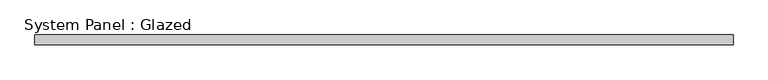
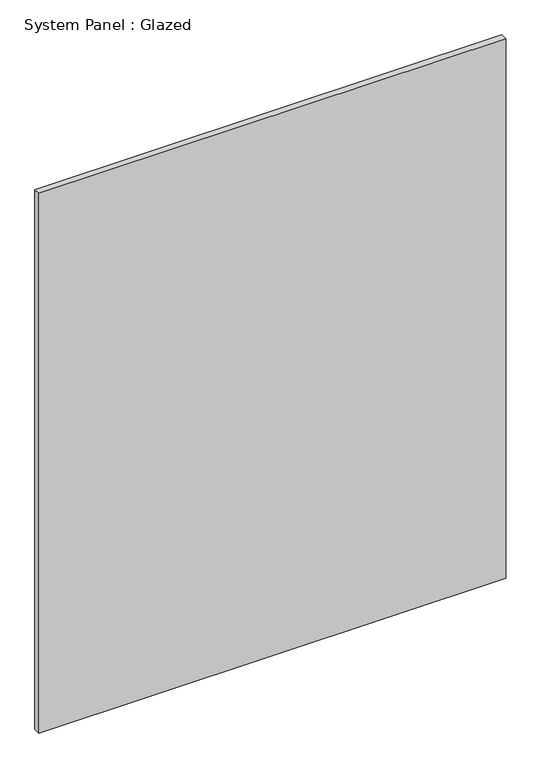
"""IFC4 building model written with IfcOpenShell, lengths in millimetres: plate geometry, System Panel : Glazed."""

import ifcopenshell
import ifcopenshell.guid

model = None  # the IFC model being written
_history = None  # IfcOwnerHistory: only IFC2X3 demands one
_inside = {}  # id of a spatial element -> (the spatial element, [elements in it])
_under = {}  # id of a project, library or spatial element -> (it, [spatial elements below it])
_declared = {}  # id of a project -> (the project, [libraries it declares])
_typed = {}  # id of a type object -> (the type object, [elements of that type])
_made_of = {}  # id of a material, layer set ... -> (it, [elements and type objects made of it])


def new_model(schema):
    """Start an empty IFC model of exactly this schema.

    Asked for "IFC4X3", IfcOpenShell would pick the latest addendum, in which some entities
    have other attributes; the version numbers below select the first issue.
    IFC2X3 requires an IfcOwnerHistory on every rooted entity: one is made here for all.
    """
    global model, _history
    if schema == "IFC4X3":
        model = ifcopenshell.file(schema_version=(4, 3, 0, 0))
    else:
        model = ifcopenshell.file(schema=schema)
    _inside.clear()
    _under.clear()
    _declared.clear()
    _typed.clear()
    _made_of.clear()
    _history = None
    if model.schema == "IFC2X3":
        org = make("IfcOrganization", Name="unknown")
        user = make(
            "IfcPersonAndOrganization",
            ThePerson=make("IfcPerson", FamilyName="unknown"),
            TheOrganization=org,
        )
        app = make(
            "IfcApplication",
            ApplicationDeveloper=org,
            Version="unknown",
            ApplicationFullName="unknown",
            ApplicationIdentifier="unknown",
        )
        _history = make(
            "IfcOwnerHistory",
            OwningUser=user,
            OwningApplication=app,
            ChangeAction="ADDED",
            CreationDate=0,
        )
    return model


def make(cls, **values):
    """One entity of the class cls with the attributes given. An attribute that is None is left unset."""
    return model.create_entity(
        cls, **{name: value for name, value in values.items() if value is not None}
    )


def rooted(cls, **values):
    """An entity with a GlobalId (a new one), such as an element, a storey or a relation."""
    return make(cls, GlobalId=ifcopenshell.guid.new(), OwnerHistory=_history, **values)


def si_unit(unit_type, name, prefix=None):
    """IfcSIUnit, for example si_unit("LENGTHUNIT", "METRE", prefix="MILLI")."""
    return make("IfcSIUnit", UnitType=unit_type, Prefix=prefix, Name=name)


def assignment(units):
    """IfcUnitAssignment: the units of a project."""
    return None if units is None else make("IfcUnitAssignment", Units=units)


def point(xyz):
    """IfcCartesianPoint."""
    return None if xyz is None else make("IfcCartesianPoint", Coordinates=xyz)


def direction(xyz):
    """IfcDirection."""
    return None if xyz is None else make("IfcDirection", DirectionRatios=xyz)


def frame(location, z_axis=None, x_axis=None):
    """IfcAxis2Placement3D, a coordinate frame: its origin and axes. An axis left out is left unset."""
    return make(
        "IfcAxis2Placement3D",
        Location=point(location),
        Axis=direction(z_axis),
        RefDirection=direction(x_axis),
    )


def origin():
    """The frame at (0, 0, 0) with its axes left unset."""
    return frame((0.0, 0.0, 0.0))


def origin_with_axes():
    """The frame at (0, 0, 0) with the z axis (0, 0, 1) and the x axis (1, 0, 0) written out."""
    return frame((0.0, 0.0, 0.0), z_axis=(0.0, 0.0, 1.0), x_axis=(1.0, 0.0, 0.0))


def place(relative_to, where):
    """IfcLocalPlacement: puts the frame where relative to a parent placement (None: the world)."""
    return make(
        "IfcLocalPlacement", PlacementRelTo=relative_to, RelativePlacement=where
    )


def context(
    kind, dimensions, precision=None, world=None, true_north=None, identifier=None
):
    """IfcGeometricRepresentationContext, for example the 3D "Model" context."""
    return make(
        "IfcGeometricRepresentationContext",
        ContextIdentifier=identifier,
        ContextType=kind,
        CoordinateSpaceDimension=dimensions,
        Precision=precision,
        WorldCoordinateSystem=world,
        TrueNorth=true_north,
    )


def project(units=None, contexts=None):
    """IfcProject with its units and contexts."""
    return rooted(
        "IfcProject",
        Name="project",
        RepresentationContexts=contexts,
        UnitsInContext=assignment(units),
    )


def spatial(cls, under=None, at=None, **own):
    """A site, building, storey or space (cls), placed at a placement, below another one or the project."""
    s = rooted(cls, ObjectPlacement=at, **own)
    if under is not None:
        _under.setdefault(under.id(), (under, []))[1].append(s)
    return s


def polyline(points):
    """IfcPolyline through the points."""
    return make("IfcPolyline", Points=[point(p) for p in points])


def outline(outer, holes=None, kind="AREA"):
    """IfcArbitraryClosedProfileDef: a profile drawn as a closed curve; with holes, ...WithVoids."""
    if holes is None:
        return make("IfcArbitraryClosedProfileDef", ProfileType=kind, OuterCurve=outer)
    return make(
        "IfcArbitraryProfileDefWithVoids",
        ProfileType=kind,
        OuterCurve=outer,
        InnerCurves=holes,
    )


def extrude(swept, where, along, depth):
    """IfcExtrudedAreaSolid: the profile swept, set in the frame where, extruded along a direction by depth."""
    return make(
        "IfcExtrudedAreaSolid",
        SweptArea=swept,
        Position=where,
        ExtrudedDirection=direction(along),
        Depth=depth,
    )


def shape(context_of_items, identifier, shape_type, items):
    """IfcShapeRepresentation: the items that make up one representation, for example the "Body"."""
    return make(
        "IfcShapeRepresentation",
        ContextOfItems=context_of_items,
        RepresentationIdentifier=identifier,
        RepresentationType=shape_type,
        Items=items,
    )


def source(mapping_origin, context_of_items, identifier, shape_type, items):
    """IfcRepresentationMap: a shape defined once, which mapped items show again and again."""
    return make(
        "IfcRepresentationMap",
        MappingOrigin=mapping_origin,
        MappedRepresentation=shape(context_of_items, identifier, shape_type, items),
    )


def transform(
    local_origin,
    x_axis=None,
    y_axis=None,
    z_axis=None,
    scale=None,
    scale2=None,
    scale3=None,
    uniform=True,
):
    """IfcCartesianTransformationOperator3D, or its non-uniform kind. x_axis, y_axis, z_axis: its Axis1, 2, 3."""
    if uniform:
        return make(
            "IfcCartesianTransformationOperator3D",
            Axis1=direction(x_axis),
            Axis2=direction(y_axis),
            LocalOrigin=point(local_origin),
            Scale=scale,
            Axis3=direction(z_axis),
        )
    return make(
        "IfcCartesianTransformationOperator3DnonUniform",
        Axis1=direction(x_axis),
        Axis2=direction(y_axis),
        LocalOrigin=point(local_origin),
        Scale=scale,
        Axis3=direction(z_axis),
        Scale2=scale2,
        Scale3=scale3,
    )


def mapped(mapping_source, mapping_target):
    """IfcMappedItem: shows the shape of a source again, moved by a transform."""
    return make(
        "IfcMappedItem", MappingSource=mapping_source, MappingTarget=mapping_target
    )


def made_of(thing, what):
    """Note that an element or type object is made of a material, layer set ...; save() writes the relation."""
    if what is not None:
        _made_of.setdefault(what.id(), (what, []))[1].append(thing)
    return thing


def element(
    cls,
    number,
    at=None,
    inside=None,
    cuts=None,
    type_object=None,
    material=None,
    context=None,
    identifier="Body",
    shape_type=None,
    held_by="IfcProductDefinitionShape",
    body=None,
    shapes=None,
    **own,
):
    """One element of the class cls, such as IfcWall. Its Tag is "e" and its number.

    at: its placement. inside: the storey or other place that contains it. cuts: it is an
    opening in that element (IfcRelVoidsElement). A single representation is given by context,
    identifier, shape_type and body (its items); several are given by shapes. held_by: the class
    of the entity that holds the representations. save() writes the other relations.
    """
    e = rooted(cls, Tag="e%d" % number, ObjectPlacement=at, **own)
    if body is not None:
        shapes = [shape(context, identifier, shape_type, body)]
    if shapes is not None:
        e.Representation = make(held_by, Representations=shapes)
    if inside is not None:
        _inside.setdefault(inside.id(), (inside, []))[1].append(e)
    if cuts is not None:
        rooted(
            "IfcRelVoidsElement", RelatingBuildingElement=cuts, RelatedOpeningElement=e
        )
    if type_object is not None:
        _typed.setdefault(type_object.id(), (type_object, []))[1].append(e)
    return made_of(e, material)


def aggregate(whole, parts):
    """IfcRelAggregates: a whole, such as a stair, and the parts it consists of."""
    return rooted("IfcRelAggregates", RelatingObject=whole, RelatedObjects=parts)


def save(model, path):
    """Write the relations noted so far, then the file.

    IfcRelAggregates (storeys below a building ...), IfcRelContainedInSpatialStructure (elements
    in a storey), IfcRelDefinesByType, IfcRelAssociatesMaterial and IfcRelDeclares: one each for
    every whole, place, type object, material and project.
    """
    for whole, parts in _under.values():
        aggregate(whole, parts)
    for where, things in _inside.values():
        rooted(
            "IfcRelContainedInSpatialStructure",
            RelatedElements=things,
            RelatingStructure=where,
        )
    for kind, things in _typed.values():
        rooted("IfcRelDefinesByType", RelatedObjects=things, RelatingType=kind)
    for what, things in _made_of.values():
        rooted("IfcRelAssociatesMaterial", RelatedObjects=things, RelatingMaterial=what)
    for by, libraries in _declared.values():
        rooted("IfcRelDeclares", RelatingContext=by, RelatedDefinitions=libraries)
    model.write(path)


def system_panel_glazed_f186845e(model_context):
    return source(origin(), model_context, "Body", "SweptSolid", [
        extrude(outline(polyline([(879.5, -49.5), (-879.5, -49.5), (-879.5, -24.5), (879.5, -24.5), (879.5, -49.5)])), origin_with_axes(), (0.0, 0.0, 1.0), 2150.0),
    ])


if __name__ == "__main__":
    model = new_model("IFC4")
    model_context = context("Model", 3, world=origin())
    ifc_project = project(units=[si_unit("LENGTHUNIT", "METRE", prefix="MILLI")], contexts=[model_context])
    site = spatial("IfcSite", under=ifc_project)
    building = spatial("IfcBuilding", under=site)
    placement = place(None, origin())
    system_panel_glazed_shape = system_panel_glazed_f186845e(model_context)
    element("IfcPlate", 1, ObjectType="System Panel : Glazed", at=placement, inside=building, context=model_context, shape_type="MappedRepresentation", body=[
        mapped(system_panel_glazed_shape, transform((0.0, 0.0, 0.0), x_axis=(1.0, 0.0, 0.0), y_axis=(0.0, 1.0, 0.0), z_axis=(0.0, 0.0, 1.0))),
    ])
    save(model, "model.ifc")

# Revit data of these elements
# Type "System Panel : Glazed"
#   Keynote = "H11"
#   Construction Type Id = "GSP4R"
#   Analytic Construction = "1/8 in Pilkington single glazing"
#   Visual Light Transmittance = 0.9
#   Solar Heat Gain Coefficient = 0.86
#   Heat Transfer Coefficient (U) = 6.7069 W/(m²·K)
# Element 1 (IfcPlate, "System Panel : Glazed")
#   Materials on its faces: "Glass"
# Materials
#   "Glass": class "Glass", colour RGB 0 128 192, transparency 0.9, Description = "Soda Lime Glass", Cost = 0
